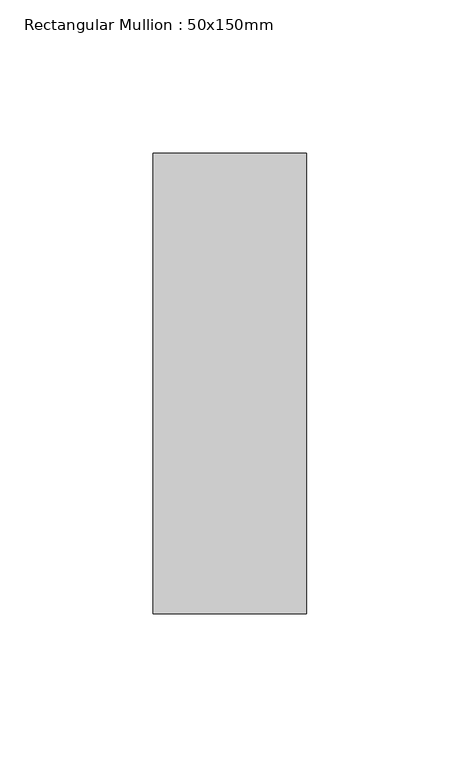
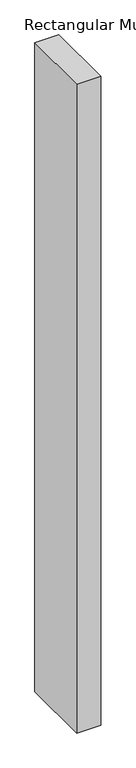
"""IFC4 building model written with IfcOpenShell, lengths in millimetres: member geometry, Rectangular Mullion : 50x150mm."""

import ifcopenshell
import ifcopenshell.guid

model = None  # the IFC model being written
_history = None  # IfcOwnerHistory: only IFC2X3 demands one
_inside = {}  # id of a spatial element -> (the spatial element, [elements in it])
_under = {}  # id of a project, library or spatial element -> (it, [spatial elements below it])
_declared = {}  # id of a project -> (the project, [libraries it declares])
_typed = {}  # id of a type object -> (the type object, [elements of that type])
_made_of = {}  # id of a material, layer set ... -> (it, [elements and type objects made of it])


def new_model(schema):
    """Start an empty IFC model of exactly this schema.

    Asked for "IFC4X3", IfcOpenShell would pick the latest addendum, in which some entities
    have other attributes; the version numbers below select the first issue.
    IFC2X3 requires an IfcOwnerHistory on every rooted entity: one is made here for all.
    """
    global model, _history
    if schema == "IFC4X3":
        model = ifcopenshell.file(schema_version=(4, 3, 0, 0))
    else:
        model = ifcopenshell.file(schema=schema)
    _inside.clear()
    _under.clear()
    _declared.clear()
    _typed.clear()
    _made_of.clear()
    _history = None
    if model.schema == "IFC2X3":
        org = make("IfcOrganization", Name="unknown")
        user = make(
            "IfcPersonAndOrganization",
            ThePerson=make("IfcPerson", FamilyName="unknown"),
            TheOrganization=org,
        )
        app = make(
            "IfcApplication",
            ApplicationDeveloper=org,
            Version="unknown",
            ApplicationFullName="unknown",
            ApplicationIdentifier="unknown",
        )
        _history = make(
            "IfcOwnerHistory",
            OwningUser=user,
            OwningApplication=app,
            ChangeAction="ADDED",
            CreationDate=0,
        )
    return model


def make(cls, **values):
    """One entity of the class cls with the attributes given. An attribute that is None is left unset."""
    return model.create_entity(
        cls, **{name: value for name, value in values.items() if value is not None}
    )


def rooted(cls, **values):
    """An entity with a GlobalId (a new one), such as an element, a storey or a relation."""
    return make(cls, GlobalId=ifcopenshell.guid.new(), OwnerHistory=_history, **values)


def si_unit(unit_type, name, prefix=None):
    """IfcSIUnit, for example si_unit("LENGTHUNIT", "METRE", prefix="MILLI")."""
    return make("IfcSIUnit", UnitType=unit_type, Prefix=prefix, Name=name)


def assignment(units):
    """IfcUnitAssignment: the units of a project."""
    return None if units is None else make("IfcUnitAssignment", Units=units)


def point(xyz):
    """IfcCartesianPoint."""
    return None if xyz is None else make("IfcCartesianPoint", Coordinates=xyz)


def direction(xyz):
    """IfcDirection."""
    return None if xyz is None else make("IfcDirection", DirectionRatios=xyz)


def frame(location, z_axis=None, x_axis=None):
    """IfcAxis2Placement3D, a coordinate frame: its origin and axes. An axis left out is left unset."""
    return make(
        "IfcAxis2Placement3D",
        Location=point(location),
        Axis=direction(z_axis),
        RefDirection=direction(x_axis),
    )


def origin():
    """The frame at (0, 0, 0) with its axes left unset."""
    return frame((0.0, 0.0, 0.0))


def place(relative_to, where):
    """IfcLocalPlacement: puts the frame where relative to a parent placement (None: the world)."""
    return make(
        "IfcLocalPlacement", PlacementRelTo=relative_to, RelativePlacement=where
    )


def context(
    kind, dimensions, precision=None, world=None, true_north=None, identifier=None
):
    """IfcGeometricRepresentationContext, for example the 3D "Model" context."""
    return make(
        "IfcGeometricRepresentationContext",
        ContextIdentifier=identifier,
        ContextType=kind,
        CoordinateSpaceDimension=dimensions,
        Precision=precision,
        WorldCoordinateSystem=world,
        TrueNorth=true_north,
    )


def project(units=None, contexts=None):
    """IfcProject with its units and contexts."""
    return rooted(
        "IfcProject",
        Name="project",
        RepresentationContexts=contexts,
        UnitsInContext=assignment(units),
    )


def spatial(cls, under=None, at=None, **own):
    """A site, building, storey or space (cls), placed at a placement, below another one or the project."""
    s = rooted(cls, ObjectPlacement=at, **own)
    if under is not None:
        _under.setdefault(under.id(), (under, []))[1].append(s)
    return s


def polyline(points):
    """IfcPolyline through the points."""
    return make("IfcPolyline", Points=[point(p) for p in points])


def outline(outer, holes=None, kind="AREA"):
    """IfcArbitraryClosedProfileDef: a profile drawn as a closed curve; with holes, ...WithVoids."""
    if holes is None:
        return make("IfcArbitraryClosedProfileDef", ProfileType=kind, OuterCurve=outer)
    return make(
        "IfcArbitraryProfileDefWithVoids",
        ProfileType=kind,
        OuterCurve=outer,
        InnerCurves=holes,
    )


def extrude(swept, where, along, depth):
    """IfcExtrudedAreaSolid: the profile swept, set in the frame where, extruded along a direction by depth."""
    return make(
        "IfcExtrudedAreaSolid",
        SweptArea=swept,
        Position=where,
        ExtrudedDirection=direction(along),
        Depth=depth,
    )


def shape(context_of_items, identifier, shape_type, items):
    """IfcShapeRepresentation: the items that make up one representation, for example the "Body"."""
    return make(
        "IfcShapeRepresentation",
        ContextOfItems=context_of_items,
        RepresentationIdentifier=identifier,
        RepresentationType=shape_type,
        Items=items,
    )


def source(mapping_origin, context_of_items, identifier, shape_type, items):
    """IfcRepresentationMap: a shape defined once, which mapped items show again and again."""
    return make(
        "IfcRepresentationMap",
        MappingOrigin=mapping_origin,
        MappedRepresentation=shape(context_of_items, identifier, shape_type, items),
    )


def transform(
    local_origin,
    x_axis=None,
    y_axis=None,
    z_axis=None,
    scale=None,
    scale2=None,
    scale3=None,
    uniform=True,
):
    """IfcCartesianTransformationOperator3D, or its non-uniform kind. x_axis, y_axis, z_axis: its Axis1, 2, 3."""
    if uniform:
        return make(
            "IfcCartesianTransformationOperator3D",
            Axis1=direction(x_axis),
            Axis2=direction(y_axis),
            LocalOrigin=point(local_origin),
            Scale=scale,
            Axis3=direction(z_axis),
        )
    return make(
        "IfcCartesianTransformationOperator3DnonUniform",
        Axis1=direction(x_axis),
        Axis2=direction(y_axis),
        LocalOrigin=point(local_origin),
        Scale=scale,
        Axis3=direction(z_axis),
        Scale2=scale2,
        Scale3=scale3,
    )


def mapped(mapping_source, mapping_target):
    """IfcMappedItem: shows the shape of a source again, moved by a transform."""
    return make(
        "IfcMappedItem", MappingSource=mapping_source, MappingTarget=mapping_target
    )


def made_of(thing, what):
    """Note that an element or type object is made of a material, layer set ...; save() writes the relation."""
    if what is not None:
        _made_of.setdefault(what.id(), (what, []))[1].append(thing)
    return thing


def element(
    cls,
    number,
    at=None,
    inside=None,
    cuts=None,
    type_object=None,
    material=None,
    context=None,
    identifier="Body",
    shape_type=None,
    held_by="IfcProductDefinitionShape",
    body=None,
    shapes=None,
    **own,
):
    """One element of the class cls, such as IfcWall. Its Tag is "e" and its number.

    at: its placement. inside: the storey or other place that contains it. cuts: it is an
    opening in that element (IfcRelVoidsElement). A single representation is given by context,
    identifier, shape_type and body (its items); several are given by shapes. held_by: the class
    of the entity that holds the representations. save() writes the other relations.
    """
    e = rooted(cls, Tag="e%d" % number, ObjectPlacement=at, **own)
    if body is not None:
        shapes = [shape(context, identifier, shape_type, body)]
    if shapes is not None:
        e.Representation = make(held_by, Representations=shapes)
    if inside is not None:
        _inside.setdefault(inside.id(), (inside, []))[1].append(e)
    if cuts is not None:
        rooted(
            "IfcRelVoidsElement", RelatingBuildingElement=cuts, RelatedOpeningElement=e
        )
    if type_object is not None:
        _typed.setdefault(type_object.id(), (type_object, []))[1].append(e)
    return made_of(e, material)


def aggregate(whole, parts):
    """IfcRelAggregates: a whole, such as a stair, and the parts it consists of."""
    return rooted("IfcRelAggregates", RelatingObject=whole, RelatedObjects=parts)


def save(model, path):
    """Write the relations noted so far, then the file.

    IfcRelAggregates (storeys below a building ...), IfcRelContainedInSpatialStructure (elements
    in a storey), IfcRelDefinesByType, IfcRelAssociatesMaterial and IfcRelDeclares: one each for
    every whole, place, type object, material and project.
    """
    for whole, parts in _under.values():
        aggregate(whole, parts)
    for where, things in _inside.values():
        rooted(
            "IfcRelContainedInSpatialStructure",
            RelatedElements=things,
            RelatingStructure=where,
        )
    for kind, things in _typed.values():
        rooted("IfcRelDefinesByType", RelatedObjects=things, RelatingType=kind)
    for what, things in _made_of.values():
        rooted("IfcRelAssociatesMaterial", RelatedObjects=things, RelatingMaterial=what)
    for by, libraries in _declared.values():
        rooted("IfcRelDeclares", RelatingContext=by, RelatedDefinitions=libraries)
    model.write(path)


def rectangular_mullion_50x150mm_1f4d75dd(model_context):
    return source(origin(), model_context, "Body", "SweptSolid", [
        extrude(outline(polyline([(25.0, 75.0), (25.0, -75.0), (-25.0, -75.0), (-25.0, 75.0), (25.0, 75.0)])), frame((0.0, 0.0, -1425.0), z_axis=(0.0, 0.0, 1.0), x_axis=(1.0, 0.0, 0.0)), (0.0, 0.0, 1.0), 1425.0),
    ])


if __name__ == "__main__":
    model = new_model("IFC4")
    model_context = context("Model", 3, world=origin())
    ifc_project = project(units=[si_unit("LENGTHUNIT", "METRE", prefix="MILLI")], contexts=[model_context])
    site = spatial("IfcSite", under=ifc_project)
    building = spatial("IfcBuilding", under=site)
    placement = place(None, origin())
    rectangular_mullion_50x150mm_shape = rectangular_mullion_50x150mm_1f4d75dd(model_context)
    element("IfcMember", 1, ObjectType="Rectangular Mullion : 50x150mm", at=placement, inside=building, context=model_context, shape_type="MappedRepresentation", body=[
        mapped(rectangular_mullion_50x150mm_shape, transform((0.0, 0.0, 0.0), x_axis=(1.0, 0.0, 0.0), y_axis=(0.0, 1.0, 0.0), z_axis=(0.0, 0.0, 1.0))),
    ])
    save(model, "model.ifc")

# Revit data of these elements
# Project information
#   Project Issue Date = "Issue Date"
#   Project Status = "Project Status"
#   Client Name = "Owner"
#   Project Address = "Enter address here"
#   Project Name = "Project Name"
#   Project Number = "Project Number"
# Type "Rectangular Mullion : 50x150mm"
#   Keynote = "H11"
#   built-in parameter 1007304 = 0.492126 (stored number, unit not read)
#   built-in parameter 1007301 = 0.082021 (stored number, unit not read)
#   built-in parameter 1007300 = 0.082021 (stored number, unit not read)
# Element 1 (IfcMember, "Rectangular Mullion : 50x150mm")
#   Materials on its faces: "Aluminium"
# Materials
#   "Aluminium": class "Metal", colour RGB 247 247 247, transparency 0, Description = "Aluminium 6061", Cost = 0
